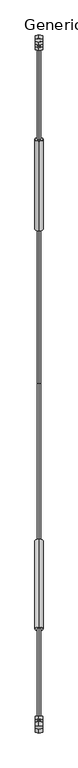
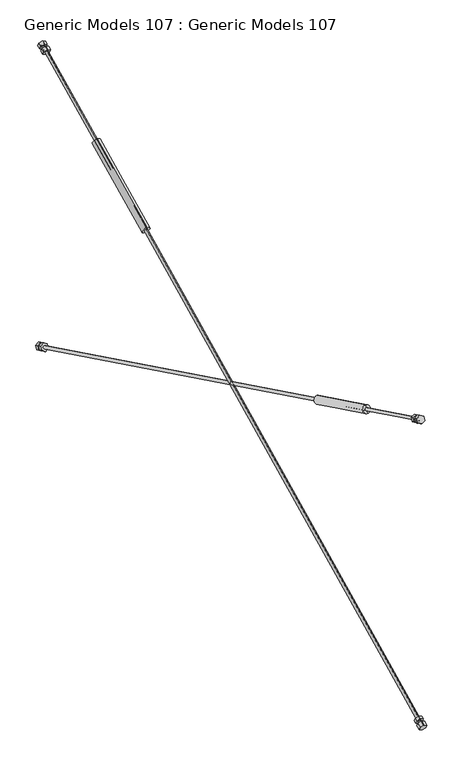
"""IFC4 building model written with IfcOpenShell, lengths in millimetres: proxy geometry, Generic Models 107 : Generic Models 107."""

import ifcopenshell
import ifcopenshell.guid

model = None  # the IFC model being written
_history = None  # IfcOwnerHistory: only IFC2X3 demands one
_inside = {}  # id of a spatial element -> (the spatial element, [elements in it])
_under = {}  # id of a project, library or spatial element -> (it, [spatial elements below it])
_declared = {}  # id of a project -> (the project, [libraries it declares])
_typed = {}  # id of a type object -> (the type object, [elements of that type])
_made_of = {}  # id of a material, layer set ... -> (it, [elements and type objects made of it])


def new_model(schema):
    """Start an empty IFC model of exactly this schema.

    Asked for "IFC4X3", IfcOpenShell would pick the latest addendum, in which some entities
    have other attributes; the version numbers below select the first issue.
    IFC2X3 requires an IfcOwnerHistory on every rooted entity: one is made here for all.
    """
    global model, _history
    if schema == "IFC4X3":
        model = ifcopenshell.file(schema_version=(4, 3, 0, 0))
    else:
        model = ifcopenshell.file(schema=schema)
    _inside.clear()
    _under.clear()
    _declared.clear()
    _typed.clear()
    _made_of.clear()
    _history = None
    if model.schema == "IFC2X3":
        org = make("IfcOrganization", Name="unknown")
        user = make(
            "IfcPersonAndOrganization",
            ThePerson=make("IfcPerson", FamilyName="unknown"),
            TheOrganization=org,
        )
        app = make(
            "IfcApplication",
            ApplicationDeveloper=org,
            Version="unknown",
            ApplicationFullName="unknown",
            ApplicationIdentifier="unknown",
        )
        _history = make(
            "IfcOwnerHistory",
            OwningUser=user,
            OwningApplication=app,
            ChangeAction="ADDED",
            CreationDate=0,
        )
    return model


def make(cls, **values):
    """One entity of the class cls with the attributes given. An attribute that is None is left unset."""
    return model.create_entity(
        cls, **{name: value for name, value in values.items() if value is not None}
    )


def rooted(cls, **values):
    """An entity with a GlobalId (a new one), such as an element, a storey or a relation."""
    return make(cls, GlobalId=ifcopenshell.guid.new(), OwnerHistory=_history, **values)


def si_unit(unit_type, name, prefix=None):
    """IfcSIUnit, for example si_unit("LENGTHUNIT", "METRE", prefix="MILLI")."""
    return make("IfcSIUnit", UnitType=unit_type, Prefix=prefix, Name=name)


def assignment(units):
    """IfcUnitAssignment: the units of a project."""
    return None if units is None else make("IfcUnitAssignment", Units=units)


def point(xyz):
    """IfcCartesianPoint."""
    return None if xyz is None else make("IfcCartesianPoint", Coordinates=xyz)


def direction(xyz):
    """IfcDirection."""
    return None if xyz is None else make("IfcDirection", DirectionRatios=xyz)


def frame(location, z_axis=None, x_axis=None):
    """IfcAxis2Placement3D, a coordinate frame: its origin and axes. An axis left out is left unset."""
    return make(
        "IfcAxis2Placement3D",
        Location=point(location),
        Axis=direction(z_axis),
        RefDirection=direction(x_axis),
    )


def origin():
    """The frame at (0, 0, 0) with its axes left unset."""
    return frame((0.0, 0.0, 0.0))


def place(relative_to, where):
    """IfcLocalPlacement: puts the frame where relative to a parent placement (None: the world)."""
    return make(
        "IfcLocalPlacement", PlacementRelTo=relative_to, RelativePlacement=where
    )


def context(
    kind, dimensions, precision=None, world=None, true_north=None, identifier=None
):
    """IfcGeometricRepresentationContext, for example the 3D "Model" context."""
    return make(
        "IfcGeometricRepresentationContext",
        ContextIdentifier=identifier,
        ContextType=kind,
        CoordinateSpaceDimension=dimensions,
        Precision=precision,
        WorldCoordinateSystem=world,
        TrueNorth=true_north,
    )


def project(units=None, contexts=None):
    """IfcProject with its units and contexts."""
    return rooted(
        "IfcProject",
        Name="project",
        RepresentationContexts=contexts,
        UnitsInContext=assignment(units),
    )


def spatial(cls, under=None, at=None, **own):
    """A site, building, storey or space (cls), placed at a placement, below another one or the project."""
    s = rooted(cls, ObjectPlacement=at, **own)
    if under is not None:
        _under.setdefault(under.id(), (under, []))[1].append(s)
    return s


def polyline(points):
    """IfcPolyline through the points."""
    return make("IfcPolyline", Points=[point(p) for p in points])


def circle_curve(where, radius):
    """IfcCircle in the frame where."""
    return make("IfcCircle", Position=where, Radius=radius)


def outline(outer, holes=None, kind="AREA"):
    """IfcArbitraryClosedProfileDef: a profile drawn as a closed curve; with holes, ...WithVoids."""
    if holes is None:
        return make("IfcArbitraryClosedProfileDef", ProfileType=kind, OuterCurve=outer)
    return make(
        "IfcArbitraryProfileDefWithVoids",
        ProfileType=kind,
        OuterCurve=outer,
        InnerCurves=holes,
    )


def extrude(swept, where, along, depth):
    """IfcExtrudedAreaSolid: the profile swept, set in the frame where, extruded along a direction by depth."""
    return make(
        "IfcExtrudedAreaSolid",
        SweptArea=swept,
        Position=where,
        ExtrudedDirection=direction(along),
        Depth=depth,
    )


def shape(context_of_items, identifier, shape_type, items):
    """IfcShapeRepresentation: the items that make up one representation, for example the "Body"."""
    return make(
        "IfcShapeRepresentation",
        ContextOfItems=context_of_items,
        RepresentationIdentifier=identifier,
        RepresentationType=shape_type,
        Items=items,
    )


def source(mapping_origin, context_of_items, identifier, shape_type, items):
    """IfcRepresentationMap: a shape defined once, which mapped items show again and again."""
    return make(
        "IfcRepresentationMap",
        MappingOrigin=mapping_origin,
        MappedRepresentation=shape(context_of_items, identifier, shape_type, items),
    )


def transform(
    local_origin,
    x_axis=None,
    y_axis=None,
    z_axis=None,
    scale=None,
    scale2=None,
    scale3=None,
    uniform=True,
):
    """IfcCartesianTransformationOperator3D, or its non-uniform kind. x_axis, y_axis, z_axis: its Axis1, 2, 3."""
    if uniform:
        return make(
            "IfcCartesianTransformationOperator3D",
            Axis1=direction(x_axis),
            Axis2=direction(y_axis),
            LocalOrigin=point(local_origin),
            Scale=scale,
            Axis3=direction(z_axis),
        )
    return make(
        "IfcCartesianTransformationOperator3DnonUniform",
        Axis1=direction(x_axis),
        Axis2=direction(y_axis),
        LocalOrigin=point(local_origin),
        Scale=scale,
        Axis3=direction(z_axis),
        Scale2=scale2,
        Scale3=scale3,
    )


def mapped(mapping_source, mapping_target):
    """IfcMappedItem: shows the shape of a source again, moved by a transform."""
    return make(
        "IfcMappedItem", MappingSource=mapping_source, MappingTarget=mapping_target
    )


def made_of(thing, what):
    """Note that an element or type object is made of a material, layer set ...; save() writes the relation."""
    if what is not None:
        _made_of.setdefault(what.id(), (what, []))[1].append(thing)
    return thing


def element(
    cls,
    number,
    at=None,
    inside=None,
    cuts=None,
    type_object=None,
    material=None,
    context=None,
    identifier="Body",
    shape_type=None,
    held_by="IfcProductDefinitionShape",
    body=None,
    shapes=None,
    **own,
):
    """One element of the class cls, such as IfcWall. Its Tag is "e" and its number.

    at: its placement. inside: the storey or other place that contains it. cuts: it is an
    opening in that element (IfcRelVoidsElement). A single representation is given by context,
    identifier, shape_type and body (its items); several are given by shapes. held_by: the class
    of the entity that holds the representations. save() writes the other relations.
    """
    e = rooted(cls, Tag="e%d" % number, ObjectPlacement=at, **own)
    if body is not None:
        shapes = [shape(context, identifier, shape_type, body)]
    if shapes is not None:
        e.Representation = make(held_by, Representations=shapes)
    if inside is not None:
        _inside.setdefault(inside.id(), (inside, []))[1].append(e)
    if cuts is not None:
        rooted(
            "IfcRelVoidsElement", RelatingBuildingElement=cuts, RelatedOpeningElement=e
        )
    if type_object is not None:
        _typed.setdefault(type_object.id(), (type_object, []))[1].append(e)
    return made_of(e, material)


def aggregate(whole, parts):
    """IfcRelAggregates: a whole, such as a stair, and the parts it consists of."""
    return rooted("IfcRelAggregates", RelatingObject=whole, RelatedObjects=parts)


def save(model, path):
    """Write the relations noted so far, then the file.

    IfcRelAggregates (storeys below a building ...), IfcRelContainedInSpatialStructure (elements
    in a storey), IfcRelDefinesByType, IfcRelAssociatesMaterial and IfcRelDeclares: one each for
    every whole, place, type object, material and project.
    """
    for whole, parts in _under.values():
        aggregate(whole, parts)
    for where, things in _inside.values():
        rooted(
            "IfcRelContainedInSpatialStructure",
            RelatedElements=things,
            RelatingStructure=where,
        )
    for kind, things in _typed.values():
        rooted("IfcRelDefinesByType", RelatedObjects=things, RelatingType=kind)
    for what, things in _made_of.values():
        rooted("IfcRelAssociatesMaterial", RelatedObjects=things, RelatingMaterial=what)
    for by, libraries in _declared.values():
        rooted("IfcRelDeclares", RelatingContext=by, RelatedDefinitions=libraries)
    model.write(path)


def plane_surface(at):
    """IfcPlane: the flat surface through the origin of the frame at, square to its z axis."""
    return make("IfcPlane", Position=at)


def cylinder_surface(at, radius):
    """IfcCylindricalSurface: all points at the distance radius from the z axis of the frame at."""
    return make("IfcCylindricalSurface", Position=at, Radius=radius)


def revolved_surface(curve, axis_point, axis_direction):
    """IfcSurfaceOfRevolution: the curve turned about the line through axis_point along axis_direction."""
    return make(
        "IfcSurfaceOfRevolution",
        SweptCurve=make("IfcArbitraryOpenProfileDef", ProfileType="CURVE", Curve=curve),
        AxisPosition=make("IfcAxis1Placement", Location=point(axis_point), Axis=direction(axis_direction)),
    )


def advanced_brep(points, edges, surfaces, faces):
    """IfcAdvancedBrep: a solid bounded by faces that lie on surfaces and meet in shared edges.

    An edge is (start, end): straight between two places in points (the first is 0);
    or (start, end, curve); or (start, end, curve, False) where it runs against its curve.
    A face is (place in surfaces, loops), or (place, loops, False) where it looks against
    its surface's normal. A loop lists edges by number (the first is 1), with a minus sign
    where the edge is run from its end to its start. The first loop is the outer one.
    """
    corners = [point(p) for p in points]
    vertices = [make("IfcVertexPoint", VertexGeometry=c) for c in corners]
    made = []
    for start, end, *more in edges:
        made.append(
            make(
                "IfcEdgeCurve",
                EdgeStart=vertices[start],
                EdgeEnd=vertices[end],
                EdgeGeometry=more[0] if more else make("IfcPolyline", Points=[corners[start], corners[end]]),
                SameSense=more[1] if len(more) > 1 else True,
            )
        )
    hull = []
    for where, loops, *sense in faces:
        bounds = []
        for j, loop in enumerate(loops):
            ring = [make("IfcOrientedEdge", EdgeElement=made[abs(k) - 1], Orientation=k > 0) for k in loop]
            bounds.append(
                make(
                    "IfcFaceOuterBound" if j == 0 else "IfcFaceBound",
                    Bound=make("IfcEdgeLoop", EdgeList=ring),
                    Orientation=True,
                )
            )
        hull.append(make("IfcAdvancedFace", Bounds=bounds, FaceSurface=surfaces[where], SameSense=sense[0] if sense else True))
    return make("IfcAdvancedBrep", Outer=make("IfcClosedShell", CfsFaces=hull))


def generic_models_107_generic_models_107_dc32012f(model_context):
    return source(origin(), model_context, "Body", "SolidModel", [
        extrude(outline(polyline([(0.0, 0.0), (25.4000001, 0.0), (38.1000001, -21.9970452), (25.4000001, -43.9940905), (0.0, -43.9940905), (-12.7, -21.9970452), (0.0, 0.0)])), frame((32011.8428836, 35153.3160534, 266495.1297709), z_axis=(0.0, -0.8982997891031171, 0.43938307761826173), x_axis=(0.0, -0.43938307761826173, -0.8982997891031171)), (0.0, 0.0, 1.0), 22.0707608),
        extrude(outline(polyline([(0.0, 0.0), (25.4000001, 0.0), (38.1000001, -21.9970452), (25.4000001, -43.9940905), (0.0, -43.9940905), (-12.7, -21.9970452), (0.0, 0.0)])), frame((32011.8428836, 35186.716913, 266478.7924939), z_axis=(0.0, -0.898299789103117, 0.43938307761826173), x_axis=(0.0, -0.43938307761826173, -0.898299789103117)), (0.0, 0.0, 1.0), 21.9637014),
        extrude(outline(polyline([(0.0, 0.0), (25.3999999, 0.0), (38.0999999, -21.9970452), (25.3999999, -43.9940905), (0.0, -43.9940905), (-12.7, -21.9970452), (0.0, 0.0)])), frame((32011.8428836, 30931.654853, 268560.060113), z_axis=(0.0, -0.8982997891031171, 0.43938307761826173), x_axis=(0.0, -0.43938307761826173, -0.8982997891031171)), (0.0, 0.0, 1.0), 29.8474059),
        extrude(outline(polyline([(0.0, 0.0), (25.4, 0.0), (38.1, -21.9970452), (25.4, -43.9940905), (0.0, -43.9940905), (-12.7000001, -21.9970452), (0.0, 0.0)])), frame((32011.8428836, 30966.7652004, 268542.8866786), z_axis=(0.0, -0.898299789103117, 0.43938307761826173), x_axis=(0.0, -0.43938307761826173, -0.898299789103117)), (0.0, 0.0, 1.0), 23.2103341),
        extrude(outline(polyline([(0.0, 0.0), (25.4000001, 0.0), (38.1000001, -21.9970452), (25.4000001, -43.9940905), (0.0, -43.9940905), (-12.7, -21.9970452), (0.0, 0.0)])), frame((32011.8428836, 30966.8232721, 268542.8582742), z_axis=(0.0, -0.898299789103117, 0.43938307761826173), x_axis=(0.0, -0.43938307761826173, -0.898299789103117)), (0.0, 0.0, 1.0), 23.2749803),
        extrude(outline(polyline([(0.0, 0.0), (12.6997344, -21.996585), (0.0, -43.9931701), (-25.3994686, -43.9931701), (-38.0992029, -21.996585), (-25.3994686, 0.0), (0.0, 0.0)])), frame((32011.8424234, 35099.0993943, 268541.6809718), z_axis=(0.0, 0.9016108403842673, 0.43254813894129207), x_axis=(0.0, -0.43254813894129207, 0.9016108403842673)), (0.0, 0.0, 1.0), 22.7926903),
        extrude(outline(polyline([(0.0, 0.0), (12.6997343, -21.996585), (0.0, -43.9931701), (-25.3994686, -43.9931701), (-38.0992029, -21.996585), (-25.3994686, 0.0), (0.0, 0.0)])), frame((32011.8424234, 35133.6448667, 268558.5723953), z_axis=(0.0, 0.9016108403842673, 0.43254813894129207), x_axis=(0.0, -0.43254813894129207, 0.9016108403842673)), (0.0, 0.0, 1.0), 21.3548185),
        extrude(outline(polyline([(0.0, 0.0), (12.6997344, -21.996585), (0.0, -43.9931701), (-25.3994686, -43.9931701), (-38.0992029, -21.996585), (-25.3994686, 0.0), (0.0, 0.0)])), frame((32011.8424234, 30869.4149383, 266478.8214326), z_axis=(0.0, 0.9016108403842673, 0.43254813894129207), x_axis=(0.0, -0.43254813894129207, 0.9016108403842673)), (0.0, 0.0, 1.0), 29.048698),
        extrude(outline(polyline([(0.0, 0.0), (12.6997343, -21.996585), (0.0, -43.9931701), (-25.3994687, -43.9931701), (-38.099203, -21.996585), (-25.3994687, 0.0), (0.0, 0.0)])), frame((32011.8424234, 30909.2810897, 266498.2654539), z_axis=(0.0, 0.9016108403842673, 0.43254813894129207), x_axis=(0.0, -0.43254813894129207, 0.9016108403842673)), (0.0, 0.0, 1.0), 18.2396845),
        advanced_brep(
        [(31989.8458384, 34533.8264496, 268280.4979493), (31989.8458384, 34556.0957038, 268234.8392117), (31989.8458384, 33999.7054503, 267963.4695531), (31989.8458384, 33977.436196, 268009.1282907), (31989.8458384, 34544.9610767, 268257.6685805), (31989.8458384, 33988.5708232, 267986.2989219)],
        [
            (0, 1, circle_curve(frame((31989.8458384, 34544.9610767, 268257.6685805), z_axis=(0.0, -0.8987940462991656, -0.43837114678908023), x_axis=(0.0, 0.43837114678908023, -0.8987940462991656)), 25.4)),
            (1, 2),
            (2, 3, circle_curve(frame((31989.8458384, 33988.5708232, 267986.2989219), z_axis=(0.0, 0.8987940462991656, 0.43837114678908023), x_axis=(0.0, 0.43837114678908023, -0.8987940462991656)), 25.4)),
            (3, 0),
            (1, 0, circle_curve(frame((31989.8458384, 34544.9610767, 268257.6685805), z_axis=(0.0, -0.8987940462991656, -0.43837114678908023), x_axis=(0.0, 0.43837114678908023, -0.8987940462991656)), 25.4)),
            (3, 2, circle_curve(frame((31989.8458384, 33988.5708232, 267986.2989219), z_axis=(0.0, 0.8987940462991656, 0.43837114678908023), x_axis=(0.0, 0.43837114678908023, -0.8987940462991656)), 25.4)),
            (4, 1),
            (0, 4),
            (2, 5),
            (5, 3),
        ],
        [
            cylinder_surface(frame((31989.8458384, 35167.3509481, 268561.2284036), z_axis=(0.0, 0.8987940462991656, 0.43837114678908023), x_axis=(0.0, 0.43837114678908023, -0.8987940462991656)), 25.4),
            plane_surface(frame((31989.8458384, 34544.9610767, 268257.6685805), z_axis=(0.0, 0.8987940462991656, 0.43837114678908023), x_axis=(0.0, 0.43837114678908023, -0.8987940462991656))),
            plane_surface(frame((31989.8458384, 33988.5708232, 267986.2989219), z_axis=(0.0, -0.8987940462991656, -0.43837114678908023), x_axis=(0.0, 0.43837114678908023, -0.8987940462991656))),
        ],
        [
            (0, [[1, 2, 3, 4]]),
            (0, [[5, -4, 6, -2]]),
            (1, [[7, -1, 8]]),
            (1, [[-8, -5, -7]]),
            (2, [[-3, 9, 10]]),
            (2, [[-6, -10, -9]]),
        ],
    ),
        advanced_brep(
        [(31989.8458384, 34132.8926389, 268067.2869082), (31989.8458384, 34141.2436093, 268050.1648816), (31989.8458384, 30892.4935882, 266465.6436242), (31989.8458384, 30884.1426179, 266482.7656508), (31989.8458384, 34137.0681241, 268058.7258949), (31989.8458384, 30888.3181031, 266474.2046375)],
        [
            (0, 1, circle_curve(frame((31989.8458384, 34137.0681241, 268058.7258949), z_axis=(0.0, -0.8987940462991656, -0.43837114678908023), x_axis=(0.0, 0.43837114678908023, -0.8987940462991656)), 9.525)),
            (1, 2),
            (2, 3, circle_curve(frame((31989.8458384, 30888.3181031, 266474.2046375), z_axis=(0.0, 0.8987940462991656, 0.43837114678908023), x_axis=(0.0, 0.43837114678908023, -0.8987940462991656)), 9.525)),
            (3, 0),
            (1, 0, circle_curve(frame((31989.8458384, 34137.0681241, 268058.7258949), z_axis=(0.0, -0.8987940462991656, -0.43837114678908023), x_axis=(0.0, 0.43837114678908023, -0.8987940462991656)), 9.525)),
            (3, 2, circle_curve(frame((31989.8458384, 30888.3181031, 266474.2046375), z_axis=(0.0, 0.8987940462991656, 0.43837114678908023), x_axis=(0.0, 0.43837114678908023, -0.8987940462991656)), 9.525)),
            (4, 1),
            (0, 4),
            (2, 5),
            (5, 3),
        ],
        [
            cylinder_surface(frame((31989.8458384, 35167.3509481, 268561.2284036), z_axis=(0.0, 0.8987940462991656, 0.43837114678908023), x_axis=(0.0, 0.43837114678908023, -0.8987940462991656)), 9.525),
            plane_surface(frame((31989.8458384, 34137.0681241, 268058.7258949), z_axis=(0.0, 0.8987940462991656, 0.43837114678908023), x_axis=(0.0, 0.43837114678908023, -0.8987940462991656))),
            plane_surface(frame((31989.8458384, 30888.3181031, 266474.2046375), z_axis=(0.0, -0.8987940462991656, -0.43837114678908023), x_axis=(0.0, 0.43837114678908023, -0.8987940462991656))),
        ],
        [
            (0, [[1, 2, 3, 4]]),
            (0, [[5, -4, 6, -2]]),
            (1, [[7, -1, 8]]),
            (1, [[-8, -5, -7]]),
            (2, [[-3, 9, 10]]),
            (2, [[-6, -10, -9]]),
        ],
    ),
        advanced_brep(
        [(31989.8458384, 35165.7965069, 266464.2867082), (31989.8458384, 35174.1646601, 266481.3950371), (31989.8458384, 35169.7891839, 266472.9344915), (31989.8458384, 31862.0445483, 268080.2424514), (31989.8458384, 31870.4127014, 268097.3507803), (31989.8458384, 31866.2286249, 268088.7966158)],
        [
            (0, 1, circle_curve(frame((31989.8458384, 35169.9805835, 266472.8408727), z_axis=(0.0, 0.8982997891029865, -0.4393830776185287), x_axis=(0.0, 0.4393830776185287, 0.8982997891029865)), 9.5226166)),
            (1, 2),
            (2, 0),
            (1, 0, circle_curve(frame((31989.8458384, 35169.9805835, 266472.8408727), z_axis=(0.0, 0.8982997891029865, -0.4393830776185287), x_axis=(0.0, 0.4393830776185287, 0.8982997891029865)), 9.5226166)),
            (3, 4, circle_curve(frame((31989.8458384, 31866.2286249, 268088.7966158), z_axis=(0.0, 0.8982997891029865, -0.4393830776185287), x_axis=(0.0, 0.4393830776185287, 0.8982997891029865)), 9.5226166)),
            (4, 1),
            (0, 3),
            (4, 3, circle_curve(frame((31989.8458384, 31866.2286249, 268088.7966158), z_axis=(0.0, 0.8982997891029865, -0.4393830776185287), x_axis=(0.0, 0.4393830776185287, 0.8982997891029865)), 9.5226166)),
            (5, 4),
            (3, 5),
        ],
        [
            revolved_surface(polyline([(31989.8458384, 35169.7891839, 266472.9344915), (31989.8458384, 35174.1646601, 266481.3950371)]), (31989.8458384, 30896.5140025, 268563.1106481), (0.0, -0.8982997891029865, 0.4393830776185287)),
            cylinder_surface(frame((31989.8458384, 30896.5140025, 268563.1106481), z_axis=(0.0, -0.8982997891029865, 0.4393830776185287), x_axis=(0.0, 0.4393830776185287, 0.8982997891029865)), 9.5226166),
            plane_surface(frame((31989.8458384, 31866.2286249, 268088.7966158), z_axis=(0.0, -0.8982997891029865, 0.4393830776185287), x_axis=(0.0, 0.4393830776185287, 0.8982997891029865))),
        ],
        [
            (0, [[1, 2, 3]]),
            (0, [[4, -3, -2]]),
            (1, [[5, 6, -1, 7]]),
            (1, [[8, -7, -4, -6]]),
            (2, [[9, -5, 10]]),
            (2, [[-10, -8, -9]]),
        ],
    ),
        advanced_brep(
        [(31989.8458384, 30911.5533574, 268545.1537758), (31989.8458384, 30919.9215105, 268562.2621048), (31989.8458384, 31733.5118136, 268164.3127613), (31989.8458384, 31725.1436604, 268147.2044324), (31989.8458384, 30915.5460344, 268553.8015591), (31989.8458384, 31729.327737, 268155.7585969)],
        [
            (0, 1, circle_curve(frame((31989.8458384, 30915.737434, 268553.7079403), z_axis=(0.0, 0.8982997891029865, -0.4393830776185287), x_axis=(0.0, 0.4393830776185287, 0.8982997891029865)), 9.5226166)),
            (1, 2),
            (2, 3, circle_curve(frame((31989.8458384, 31729.327737, 268155.7585969), z_axis=(0.0, -0.8982997891029865, 0.4393830776185287), x_axis=(0.0, 0.4393830776185287, 0.8982997891029865)), 9.5226166)),
            (3, 0),
            (1, 0, circle_curve(frame((31989.8458384, 30915.737434, 268553.7079403), z_axis=(0.0, 0.8982997891029865, -0.4393830776185287), x_axis=(0.0, 0.4393830776185287, 0.8982997891029865)), 9.5226166)),
            (3, 2, circle_curve(frame((31989.8458384, 31729.327737, 268155.7585969), z_axis=(0.0, -0.8982997891029865, 0.4393830776185287), x_axis=(0.0, 0.4393830776185287, 0.8982997891029865)), 9.5226166)),
            (4, 1),
            (0, 4),
            (2, 5),
            (5, 3),
        ],
        [
            cylinder_surface(frame((31989.8458384, 30896.5140025, 268563.1106481), z_axis=(0.0, -0.8982997891029865, 0.4393830776185287), x_axis=(0.0, 0.4393830776185287, 0.8982997891029865)), 9.5226166),
            revolved_surface(polyline([(31989.8458384, 30919.9215105, 268562.2621048), (31989.8458384, 30915.5460344, 268553.8015591)]), (31989.8458384, 30896.5140025, 268563.1106481), (0.0, -0.8982997891029865, 0.4393830776185287)),
            plane_surface(frame((31989.8458384, 31729.327737, 268155.7585969), z_axis=(0.0, 0.8982997891029865, -0.4393830776185287), x_axis=(0.0, 0.4393830776185287, 0.8982997891029865))),
        ],
        [
            (0, [[1, 2, 3, 4]]),
            (0, [[5, -4, 6, -2]]),
            (1, [[7, -1, 8]]),
            (1, [[-8, -5, -7]]),
            (2, [[-3, 9, 10]]),
            (2, [[-6, -10, -9]]),
        ],
    ),
        advanced_brep(
        [(31989.8458384, 35149.6474556, 268563.1913668), (31989.8458384, 35157.9984259, 268546.0693402), (31989.8458384, 34374.9127103, 268164.1329171), (31989.8458384, 34366.56174, 268181.2549437), (31989.8458384, 35153.8229408, 268554.6303535), (31989.8458384, 34370.7372251, 268172.6939304)],
        [
            (0, 1, circle_curve(frame((31989.8458384, 35153.8229408, 268554.6303535), z_axis=(0.0, -0.8987940462991656, -0.43837114678908023), x_axis=(0.0, 0.43837114678908023, -0.8987940462991656)), 9.525)),
            (1, 2),
            (2, 3, circle_curve(frame((31989.8458384, 34370.7372251, 268172.6939304), z_axis=(0.0, 0.8987940462991656, 0.43837114678908023), x_axis=(0.0, 0.43837114678908023, -0.8987940462991656)), 9.525)),
            (3, 0),
            (1, 0, circle_curve(frame((31989.8458384, 35153.8229408, 268554.6303535), z_axis=(0.0, -0.8987940462991656, -0.43837114678908023), x_axis=(0.0, 0.43837114678908023, -0.8987940462991656)), 9.525)),
            (3, 2, circle_curve(frame((31989.8458384, 34370.7372251, 268172.6939304), z_axis=(0.0, 0.8987940462991656, 0.43837114678908023), x_axis=(0.0, 0.43837114678908023, -0.8987940462991656)), 9.525)),
            (4, 1),
            (0, 4),
            (2, 5),
            (5, 3),
        ],
        [
            cylinder_surface(frame((31989.8458384, 35167.3509481, 268561.2284036), z_axis=(0.0, 0.8987940462991656, 0.43837114678908023), x_axis=(0.0, 0.43837114678908023, -0.8987940462991656)), 9.525),
            plane_surface(frame((31989.8458384, 35153.8229408, 268554.6303535), z_axis=(0.0, 0.8987940462991656, 0.43837114678908023), x_axis=(0.0, 0.43837114678908023, -0.8987940462991656))),
            plane_surface(frame((31989.8458384, 34370.7372251, 268172.6939304), z_axis=(0.0, -0.8987940462991656, -0.43837114678908023), x_axis=(0.0, 0.43837114678908023, -0.8987940462991656))),
        ],
        [
            (0, [[1, 2, 3, 4]]),
            (0, [[5, -4, 6, -2]]),
            (1, [[7, -1, 8]]),
            (1, [[-8, -5, -7]]),
            (2, [[-3, 9, 10]]),
            (2, [[-6, -10, -9]]),
        ],
    ),
        advanced_brep(
        [(31989.8458384, 31499.0245649, 268240.1305598), (31989.8458384, 31521.3452253, 268285.7641891), (31989.8458384, 32065.6276758, 268019.5407066), (31989.8458384, 32043.3070155, 267973.9070773), (31989.8458384, 31510.1848951, 268262.9473745), (31989.8458384, 32054.4673457, 267996.7238919)],
        [
            (0, 1, circle_curve(frame((31989.8458384, 31510.1848951, 268262.9473745), z_axis=(0.0, 0.8982997891029865, -0.4393830776185287), x_axis=(0.0, 0.4393830776185287, 0.8982997891029865)), 25.4)),
            (1, 2),
            (2, 3, circle_curve(frame((31989.8458384, 32054.4673457, 267996.7238919), z_axis=(0.0, -0.8982997891029865, 0.4393830776185287), x_axis=(0.0, 0.4393830776185287, 0.8982997891029865)), 25.4)),
            (3, 0),
            (1, 0, circle_curve(frame((31989.8458384, 31510.1848951, 268262.9473745), z_axis=(0.0, 0.8982997891029865, -0.4393830776185287), x_axis=(0.0, 0.4393830776185287, 0.8982997891029865)), 25.4)),
            (3, 2, circle_curve(frame((31989.8458384, 32054.4673457, 267996.7238919), z_axis=(0.0, -0.8982997891029865, 0.4393830776185287), x_axis=(0.0, 0.4393830776185287, 0.8982997891029865)), 25.4)),
            (4, 1),
            (0, 4),
            (2, 5),
            (5, 3),
        ],
        [
            cylinder_surface(frame((31989.8458384, 30896.5140025, 268563.1106481), z_axis=(0.0, -0.8982997891029865, 0.4393830776185287), x_axis=(0.0, 0.4393830776185287, 0.8982997891029865)), 25.4),
            plane_surface(frame((31989.8458384, 31510.1848951, 268262.9473745), z_axis=(0.0, -0.8982997891029865, 0.4393830776185287), x_axis=(0.0, 0.4393830776185287, 0.8982997891029865))),
            plane_surface(frame((31989.8458384, 32054.4673457, 267996.7238919), z_axis=(0.0, 0.8982997891029865, -0.4393830776185287), x_axis=(0.0, 0.4393830776185287, 0.8982997891029865))),
        ],
        [
            (0, [[1, 2, 3, 4]]),
            (0, [[5, -4, 6, -2]]),
            (1, [[7, -1, 8]]),
            (1, [[-8, -5, -7]]),
            (2, [[-3, 9, 10]]),
            (2, [[-6, -10, -9]]),
        ],
    ),
    ])


if __name__ == "__main__":
    model = new_model("IFC4")
    model_context = context("Model", 3, world=origin())
    ifc_project = project(units=[si_unit("LENGTHUNIT", "METRE", prefix="MILLI")], contexts=[model_context])
    site = spatial("IfcSite", under=ifc_project)
    building = spatial("IfcBuilding", under=site)
    placement = place(None, origin())
    generic_models_107_generic_models_107_shape = generic_models_107_generic_models_107_dc32012f(model_context)
    element("IfcBuildingElementProxy", 1, Name="Generic Models 107 : Generic Models 107", ObjectType="Generic Models 107 : Generic Models 107", at=placement, inside=building, context=model_context, shape_type="MappedRepresentation", body=[
        mapped(generic_models_107_generic_models_107_shape, transform((0.0, 0.0, 0.0), x_axis=(1.0, 0.0, 0.0), y_axis=(0.0, 1.0, 0.0), z_axis=(0.0, 0.0, 1.0))),
    ])
    save(model, "model.ifc")

# Revit data of these elements
# Element 1 (IfcBuildingElementProxy, "Generic Models 107 : Generic Models 107")
#   Materials on its faces: "3/4\" DIA. GALV. ROD", "TURN BUCKLE"
# Materials
#   "3/4\" DIA. GALV. ROD": class "Metal", colour RGB 199 199 199, transparency 0, Description = "Carbon steel", Cost = 0
#   "TURN BUCKLE": class "Metal", colour RGB 199 199 199, transparency 0, Description = "Carbon steel", Cost = 0
